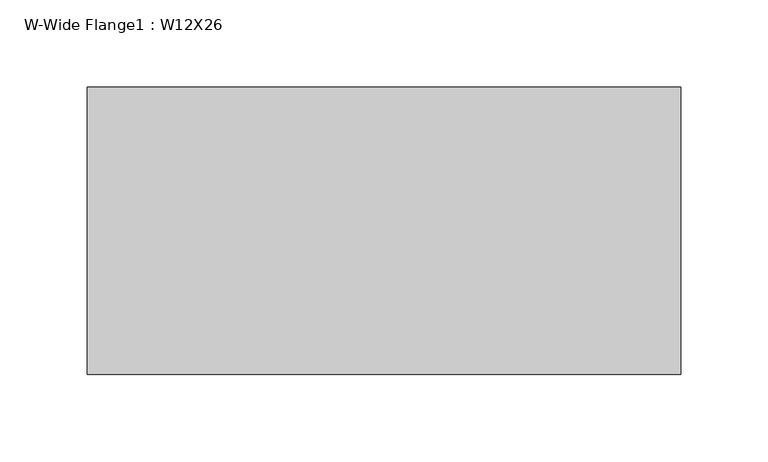
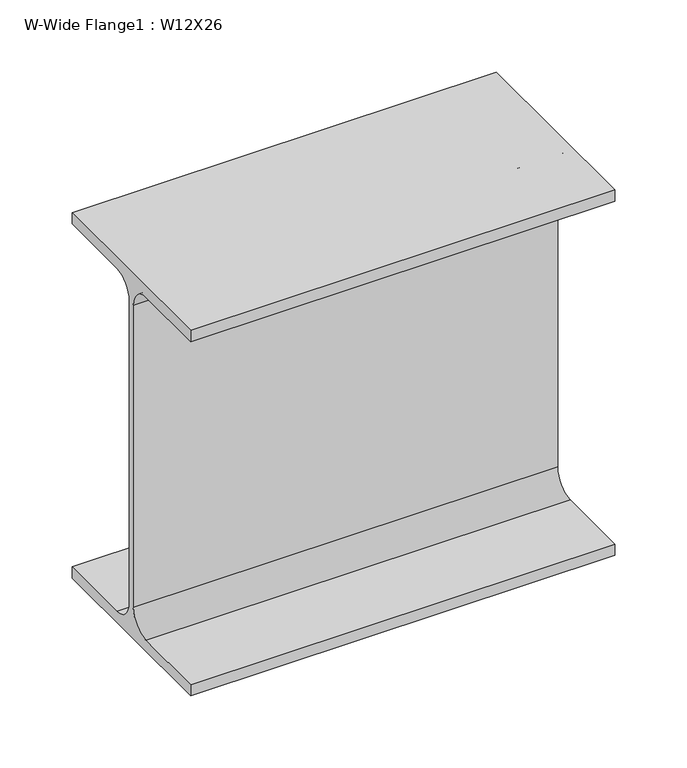
"""IFC4 building model written with IfcOpenShell, lengths in millimetres: beam geometry, W-Wide Flange1 : W12X26."""

from ifc_helpers import new_model, si_unit, point, frame, frame_2d, origin, place, context, project, spatial, polyline, circle_curve, trimmed, segment, composite_curve, outline, extrude, source, transform, mapped, element, save


def w_wide_flange1_w12x26_c1eb1bdb(model_context):
    return source(origin(), model_context, "Body", "SweptSolid", [
        extrude(outline(composite_curve([segment(polyline([(82.423, -145.288), (82.423, -154.94), (-82.423, -154.94), (-82.423, -145.288), (-20.2565, -145.288)]), True, "CONTINUOUS"), segment(trimmed(circle_curve(frame_2d((-20.2565, -127.9525)), 17.3355), [point((-20.2565, -145.288))], [point((-2.921, -127.9525))], True, "CARTESIAN"), True, "CONTINUOUS"), segment(polyline([(-2.921, -127.9525), (-2.921, 127.9525)]), True, "CONTINUOUS"), segment(trimmed(circle_curve(frame_2d((-20.2565, 127.9525)), 17.3355), [point((-2.921, 127.9525))], [point((-20.2565, 145.288))], True, "CARTESIAN"), True, "CONTINUOUS"), segment(polyline([(-20.2565, 145.288), (-82.423, 145.288), (-82.423, 154.94), (82.423, 154.94), (82.423, 145.288), (20.2565, 145.288)]), True, "CONTINUOUS"), segment(trimmed(circle_curve(frame_2d((20.2565, 127.9525)), 17.3355), [point((20.2565, 145.288))], [point((2.921, 127.9525))], True, "CARTESIAN"), True, "CONTINUOUS"), segment(polyline([(2.921, 127.9525), (2.921, -127.9525)]), True, "CONTINUOUS"), segment(trimmed(circle_curve(frame_2d((20.2565, -127.9525)), 17.3355), [point((2.921, -127.9525))], [point((20.2565, -145.288))], True, "CARTESIAN"), True, "CONTINUOUS"), segment(polyline([(20.2565, -145.288), (82.423, -145.288)]), True, "CONTINUOUS")], self_intersect=False)), frame((-157.9515116, 0.0, 0.0), z_axis=(1.0, 0.0, 0.0), x_axis=(0.0, 1.0, 0.0)), (0.0, 0.0, 1.0), 340.1667726),
    ])


if __name__ == "__main__":
    model = new_model("IFC4")
    model_context = context("Model", 3, world=origin())
    ifc_project = project(units=[si_unit("LENGTHUNIT", "METRE", prefix="MILLI")], contexts=[model_context])
    site = spatial("IfcSite", under=ifc_project)
    building = spatial("IfcBuilding", under=site)
    placement = place(None, origin())
    w_wide_flange1_w12x26_shape = w_wide_flange1_w12x26_c1eb1bdb(model_context)
    element("IfcBeam", 1, ObjectType="W-Wide Flange1 : W12X26", at=placement, inside=building, context=model_context, shape_type="MappedRepresentation", body=[
        mapped(w_wide_flange1_w12x26_shape, transform((0.0, 0.0, 0.0), x_axis=(1.0, 0.0, 0.0), y_axis=(0.0, 1.0, 0.0), z_axis=(0.0, 0.0, 1.0))),
    ])
    save(model, "model.ifc")

# Revit data of these elements
# Type "W-Wide Flange1 : W12X26"
#   Assembly Code = "B10"
#   W = 26
#   Start Extension Calculation [instance default] = 10' - 0"
#   Start Extension [instance default] = -0' - 0 1/2"
#   End Extension Calculation [instance default] = 10' - 0"
#   End Extension [instance default] = -0' - 0 1/2"
#   Length [instance default] = 5' - 0"
#   bf = 0' - 6.49"
#   d = 1' - 0.2"
#   k = 0' - 1 1/16"
#   k2 = 0' - 0.6825"
#   tf = 0' - 0.38"
#   tw = 0' - 0.23"
#   A = 0.053125 SF
#   Structural Material [instance default] = Metal - Steel - ASTM A992
# Element 1 (IfcBeam, "W-Wide Flange1 : W12X26")
#   Materials on its faces: "Metal - Steel - ASTM A992"
# Materials
#   "Metal - Steel - ASTM A992": class "Metal", colour RGB 199 199 199, transparency 0
